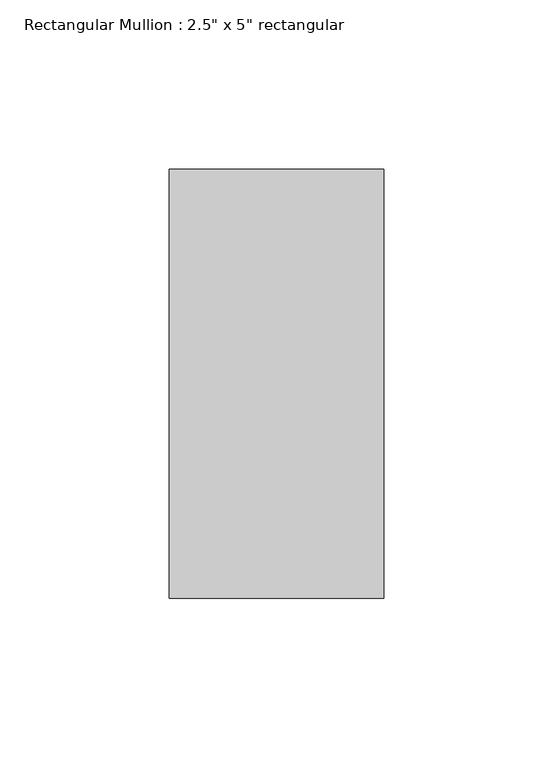
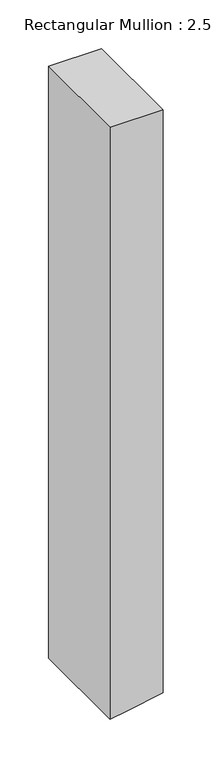
"""IFC4 building model written with IfcOpenShell, lengths in millimetres: member geometry."""

from ifc_helpers import new_model, si_unit, frame, origin, place, context, project, spatial, polyline, outline, extrude, source, transform, mapped, element, save


def member_905169d5(model_context):
    return source(origin(), model_context, "Body", "SweptSolid", [
        extrude(outline(polyline([(0.0, 31.75), (0.0, -31.75), (-744.895371, -31.75), (-741.2412869, -11.0266593), (-733.6986077, 31.75), (0.0, 31.75)])), frame((0.0, -63.5, 0.0), z_axis=(0.0, 1.0, 0.0), x_axis=(0.0, 0.0, 1.0)), (0.0, 0.0, 1.0), 127.0),
    ])


if __name__ == "__main__":
    model = new_model("IFC4")
    model_context = context("Model", 3, world=origin())
    ifc_project = project(units=[si_unit("LENGTHUNIT", "METRE", prefix="MILLI")], contexts=[model_context])
    site = spatial("IfcSite", under=ifc_project)
    building = spatial("IfcBuilding", under=site)
    placement = place(None, origin())
    member_shape = member_905169d5(model_context)
    element("IfcMember", 1, ObjectType="Rectangular Mullion : 2.5\" x 5\" rectangular", at=placement, inside=building, context=model_context, shape_type="MappedRepresentation", body=[
        mapped(member_shape, transform((0.0, 0.0, 0.0), x_axis=(1.0, 0.0, 0.0), y_axis=(0.0, 1.0, 0.0), z_axis=(0.0, 0.0, 1.0))),
    ])
    save(model, "model.ifc")

# Revit data of these elements
# Type "Rectangular Mullion : 2.5\" x 5\" rectangular"
#   built-in parameter 1007304 = 0.416667 (stored number, unit not read)
#   built-in parameter 1007301 = 0.104167 (stored number, unit not read)
#   built-in parameter 1007300 = 0.104167 (stored number, unit not read)
# Element 1 (IfcMember, "Rectangular Mullion : 2.5\" x 5\" rectangular")
#   Materials on its faces: "Black Mullions"
# Materials
#   "Black Mullions": class "Wood", colour RGB 0 0 0, transparency 0, Cost = 0
